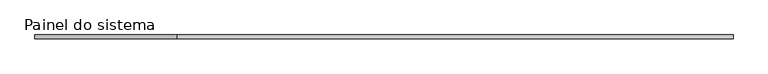
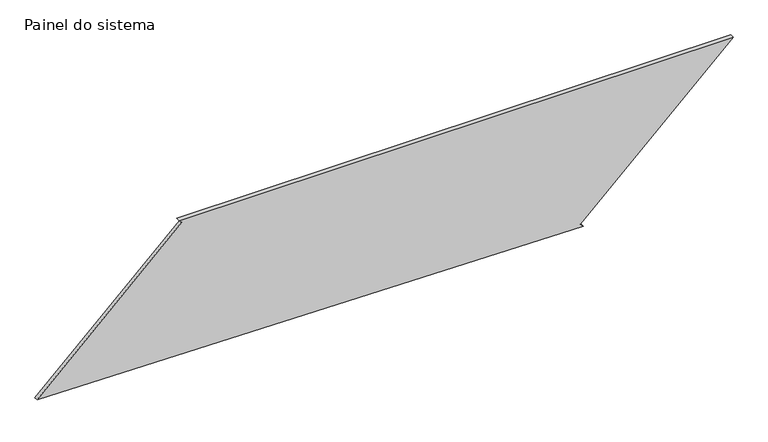
"""IFC4 building model written with IfcOpenShell, lengths in millimetres: plate geometry, Painel do sistema : Envidraçado."""

from ifc_helpers import new_model, si_unit, frame, origin, place, context, project, spatial, polyline, outline, extrude, source, transform, mapped, element, save


def painel_do_sistema_e8435c83(model_context):
    return source(origin(), model_context, "Body", "SweptSolid", [
        extrude(outline(polyline([(0.0, 1323.6464256), (18.146416, 1306.4502752), (984.9677895, 2326.6985538), (984.9677895, -1377.0794482), (966.8213735, -1359.8832978), (50.6349184, -2326.6985538), (0.0, 1323.6464256)])), frame((0.0, 24.5, 0.0), z_axis=(0.0, 1.0, 0.0), x_axis=(0.0, 0.0, 1.0)), (0.0, 0.0, 1.0), 25.0),
    ])


if __name__ == "__main__":
    model = new_model("IFC4")
    model_context = context("Model", 3, world=origin())
    ifc_project = project(units=[si_unit("LENGTHUNIT", "METRE", prefix="MILLI")], contexts=[model_context])
    site = spatial("IfcSite", under=ifc_project)
    building = spatial("IfcBuilding", under=site)
    placement = place(None, origin())
    painel_do_sistema_shape = painel_do_sistema_e8435c83(model_context)
    element("IfcPlate", 1, ObjectType="Painel do sistema : Envidraçado", at=placement, inside=building, context=model_context, shape_type="MappedRepresentation", body=[
        mapped(painel_do_sistema_shape, transform((0.0, 0.0, 0.0), x_axis=(1.0, 0.0, 0.0), y_axis=(0.0, 1.0, 0.0), z_axis=(0.0, 0.0, 1.0))),
    ])
    save(model, "model.ifc")

# Revit data of these elements
# Type "Painel do sistema : Envidraçado"
#   Construction Type Id = "GSP4R"
#   Analytic Construction = "Vidraça única Pilkington 1/8 pol"
#   Visual Light Transmittance = 0.9
#   Solar Heat Gain Coefficient = 0.86
#   Heat Transfer Coefficient (U) = 6.7069 W/(m²·K)
# Element 1 (IfcPlate, "Painel do sistema : Envidraçado")
#   Materials on its faces: "Vidro"
# Materials
#   "Vidro": class "Vidro", colour RGB 0 128 192, transparency 0.9, Description = "Vidro de sílica", Cost = 0
